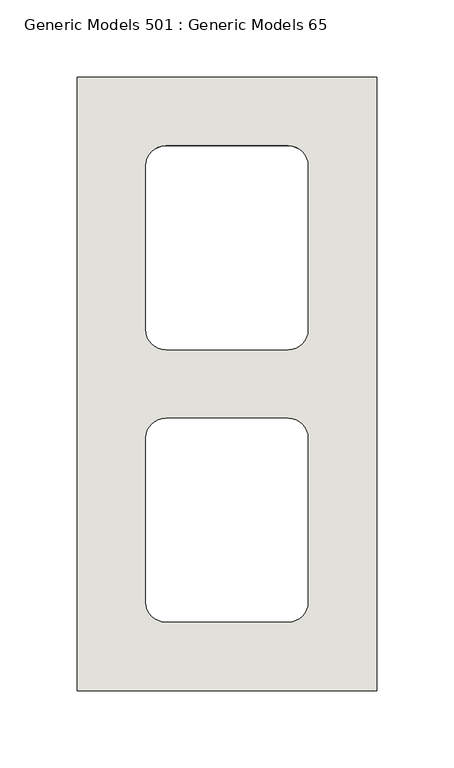
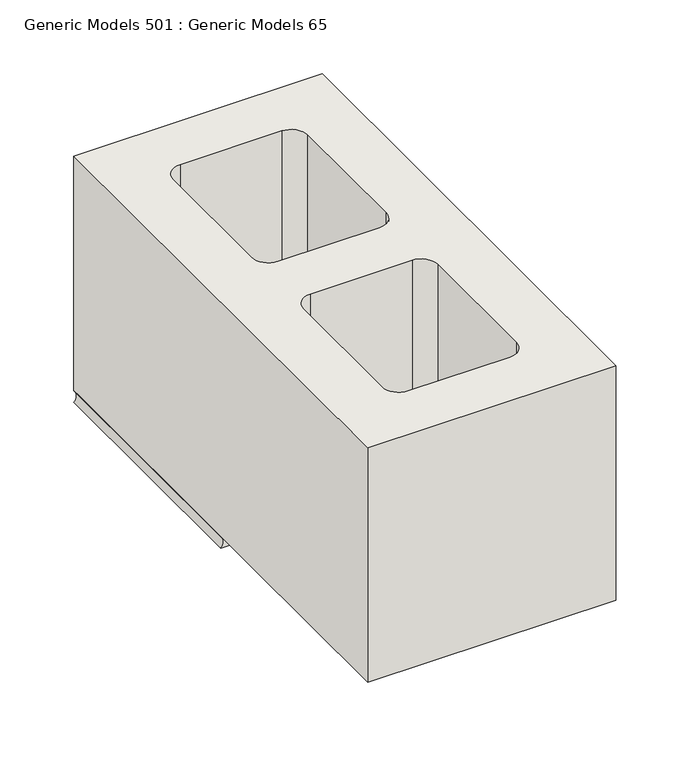
"""IFC4 building model written with IfcOpenShell, lengths in millimetres: wall geometry, Generic Models 501 : Generic Models 65."""

from ifc_helpers import new_model, si_unit, point, frame, frame_2d, origin, place, context, project, spatial, polyline, circle_curve, trimmed, segment, composite_curve, outline, extrude, source, transform, mapped, element, save
from ifc_brep_helpers import plane_surface, revolved_surface, advanced_brep


def generic_models_501_generic_models_65_e36d2a8f(model_context):
    return source(origin(), model_context, "Body", "SolidModel", [
        advanced_brep(
        [(428979.0125, 503.2375, 415.925), (428785.3375, 503.2375, 415.925), (428785.3375, 503.2375, 406.4), (428979.0125, 503.2375, 406.4), (428979.0125, 701.675, 415.925), (428979.0125, 701.675, 406.4), (428785.3375, 701.675, 406.4), (428785.3375, 701.675, 415.925), (428934.5625, 538.1625, 415.925), (428921.8625, 525.4625, 415.925), (428842.4875, 525.4625, 415.925), (428829.7875, 538.1625, 415.925), (428829.7875, 644.525, 415.925), (428842.4875, 657.225, 415.925), (428921.8625, 657.225, 415.925), (428934.5625, 644.525, 415.925), (428921.8625, 525.4625, 406.4), (428934.5625, 538.1625, 406.4), (428842.4875, 525.4625, 406.4), (428829.7875, 538.1625, 406.4), (428829.7875, 644.525, 406.4), (428842.4875, 657.225, 406.4), (428921.8625, 657.225, 406.4), (428934.5625, 644.525, 406.4)],
        [
            (0, 1),
            (1, 2, circle_curve(frame((428780.4545028, 503.2375, 411.1625), z_axis=(0.0, 1.0, 0.0), x_axis=(1.0, 0.0, 0.0)), 6.8209287)),
            (2, 3),
            (3, 0, circle_curve(frame((428983.8954972, 503.2375, 411.1625), z_axis=(0.0, 1.0, 0.0), x_axis=(-1.0, 0.0, 0.0)), 6.8209287)),
            (4, 5, circle_curve(frame((428983.8954972, 701.675, 411.1625), z_axis=(0.0, -1.0, 0.0), x_axis=(-1.0, 0.0, 0.0)), 6.8209287)),
            (5, 6),
            (6, 7, circle_curve(frame((428780.4545028, 701.675, 411.1625), z_axis=(0.0, -1.0, 0.0), x_axis=(1.0, 0.0, 0.0)), 6.8209287)),
            (7, 4),
            (0, 4),
            (7, 1),
            (8, 9, circle_curve(frame((428921.8625, 538.1625, 415.925), z_axis=(0.0, 0.0, -1.0), x_axis=(-1.0, 0.0, 0.0)), 12.7)),
            (9, 10),
            (10, 11, circle_curve(frame((428842.4875, 538.1625, 415.925), z_axis=(0.0, 0.0, -1.0), x_axis=(-1.0, 0.0, 0.0)), 12.7)),
            (11, 12),
            (12, 13, circle_curve(frame((428842.4875, 644.525, 415.925), z_axis=(0.0, 0.0, -1.0), x_axis=(-1.0, 0.0, 0.0)), 12.7)),
            (13, 14),
            (14, 15, circle_curve(frame((428921.8625, 644.525, 415.925), z_axis=(0.0, 0.0, -1.0), x_axis=(-1.0, 0.0, 0.0)), 12.7)),
            (15, 8),
            (16, 9),
            (8, 17),
            (17, 16, circle_curve(frame((428921.8625, 538.1625, 406.4), z_axis=(0.0, 0.0, -1.0), x_axis=(-1.0, 0.0, 0.0)), 12.7)),
            (16, 18),
            (18, 10),
            (18, 19, circle_curve(frame((428842.4875, 538.1625, 406.4), z_axis=(0.0, 0.0, -1.0), x_axis=(-1.0, 0.0, 0.0)), 12.7)),
            (19, 11),
            (19, 20),
            (20, 12),
            (20, 21, circle_curve(frame((428842.4875, 644.525, 406.4), z_axis=(0.0, 0.0, -1.0), x_axis=(-1.0, 0.0, 0.0)), 12.7)),
            (21, 13),
            (21, 22),
            (22, 14),
            (22, 23, circle_curve(frame((428921.8625, 644.525, 406.4), z_axis=(0.0, 0.0, -1.0), x_axis=(-1.0, 0.0, 0.0)), 12.7)),
            (23, 15),
            (23, 17),
            (6, 2),
            (5, 3),
        ],
        [
            plane_surface(frame((428882.175, 503.2375, 416.321875), z_axis=(0.0, -1.0, 0.0), x_axis=(0.0, 0.0, 1.0))),
            plane_surface(frame((428882.175, 701.675, 416.321875), z_axis=(0.0, 1.0, 0.0), x_axis=(0.0, 0.0, 1.0))),
            plane_surface(frame((428979.0125, 503.2375, 415.925), z_axis=(0.0, 0.0, 1.0), x_axis=(0.0, 1.0, 0.0))),
            revolved_surface(polyline([(428909.1625, 538.1625, 415.925), (428909.1625, 538.1625, 406.4)]), (428921.8625, 538.1625, 600.075), (0.0, 0.0, 1.0)),
            plane_surface(frame((428842.4875, 525.4625, 600.075), z_axis=(0.0, 1.0, 0.0), x_axis=(0.0, 0.0, -1.0))),
            revolved_surface(polyline([(428829.7875, 538.1625, 415.925), (428829.7875, 538.1625, 406.4)]), (428842.4875, 538.1625, 600.075), (0.0, 0.0, 1.0)),
            plane_surface(frame((428829.7875, 644.525, 600.075), z_axis=(1.0, 0.0, 0.0), x_axis=(0.0, 0.0, -1.0))),
            revolved_surface(polyline([(428829.7875, 644.525, 415.925), (428829.7875, 644.525, 406.4)]), (428842.4875, 644.525, 600.075), (0.0, 0.0, 1.0)),
            plane_surface(frame((428921.8625, 657.225, 600.075), z_axis=(0.0, -1.0, 0.0), x_axis=(0.0, 0.0, -1.0))),
            revolved_surface(polyline([(428909.1625, 644.525, 415.925), (428909.1625, 644.525, 406.4)]), (428921.8625, 644.525, 600.075), (0.0, 0.0, 1.0)),
            plane_surface(frame((428934.5625, 538.1625, 600.075), z_axis=(-1.0, 0.0, 0.0), x_axis=(0.0, 0.0, -1.0))),
            revolved_surface(polyline([(428787.2754315, 701.675, 411.1625), (428787.2754315, 503.2375, 411.1625)]), (428780.4545028, 503.2375, 411.1625), (0.0, 1.0, 0.0)),
            plane_surface(frame((428785.3375, 503.2375, 406.4), z_axis=(0.0, 0.0, -1.0), x_axis=(0.0, 1.0, 0.0))),
            revolved_surface(polyline([(428977.07456850004, 701.675, 411.1625), (428977.07456850004, 503.2375, 411.1625)]), (428983.8954972, 503.2375, 411.1625), (0.0, 1.0, 0.0)),
        ],
        [
            (0, [[1, 2, 3, 4]]),
            (1, [[5, 6, 7, 8]]),
            (2, [[-1, 9, -8, 10], [11, 12, 13, 14, 15, 16, 17, 18]]),
            (3, [[19, -11, 20, 21]]),
            (4, [[-19, 22, 23, -12]]),
            (5, [[-23, 24, 25, -13]]),
            (6, [[-25, 26, 27, -14]]),
            (7, [[-27, 28, 29, -15]]),
            (8, [[-29, 30, 31, -16]]),
            (9, [[-31, 32, 33, -17]]),
            (10, [[-33, 34, -20, -18]]),
            (11, [[-2, -10, -7, 35]]),
            (12, [[-3, -35, -6, 36], [-21, -34, -32, -30, -28, -26, -24, -22]]),
            (13, [[-4, -36, -5, -9]]),
        ],
    ),
        extrude(outline(polyline([(428979.0125, 304.8), (428785.3375, 304.8), (428785.3375, 701.675), (428979.0125, 701.675), (428979.0125, 304.8)]), holes=[composite_curve([segment(polyline([(428934.5625, 538.1625), (428934.5625, 644.525)]), True, "CONTINUOUS"), segment(trimmed(circle_curve(frame_2d((428921.8625, 644.525)), 12.7), [point((428934.5625, 644.525))], [point((428921.8625, 657.225))], True, "CARTESIAN"), True, "CONTINUOUS"), segment(polyline([(428921.8625, 657.225), (428842.4875, 657.225)]), True, "CONTINUOUS"), segment(trimmed(circle_curve(frame_2d((428842.4875, 644.525)), 12.7), [point((428842.4875, 657.225))], [point((428829.7875, 644.525))], True, "CARTESIAN"), True, "CONTINUOUS"), segment(polyline([(428829.7875, 644.525), (428829.7875, 538.1625)]), True, "CONTINUOUS"), segment(trimmed(circle_curve(frame_2d((428842.4875, 538.1625)), 12.7), [point((428829.7875, 538.1625))], [point((428842.4875, 525.4625))], True, "CARTESIAN"), True, "CONTINUOUS"), segment(polyline([(428842.4875, 525.4625), (428921.8625, 525.4625)]), True, "CONTINUOUS"), segment(trimmed(circle_curve(frame_2d((428921.8625, 538.1625)), 12.7), [point((428921.8625, 525.4625))], [point((428934.5625, 538.1625))], True, "CARTESIAN"), True, "CONTINUOUS")], self_intersect=False), composite_curve([segment(polyline([(428829.7875, 468.3125), (428829.7875, 361.95)]), True, "CONTINUOUS"), segment(trimmed(circle_curve(frame_2d((428842.4875, 361.95)), 12.7), [point((428829.7875, 361.95))], [point((428842.4875, 349.25))], True, "CARTESIAN"), True, "CONTINUOUS"), segment(polyline([(428842.4875, 349.25), (428921.8625, 349.25)]), True, "CONTINUOUS"), segment(trimmed(circle_curve(frame_2d((428921.8625, 361.95)), 12.7), [point((428921.8625, 349.25))], [point((428934.5625, 361.95))], True, "CARTESIAN"), True, "CONTINUOUS"), segment(polyline([(428934.5625, 361.95), (428934.5625, 468.3125)]), True, "CONTINUOUS"), segment(trimmed(circle_curve(frame_2d((428921.8625, 468.3125)), 12.7), [point((428934.5625, 468.3125))], [point((428921.8625, 481.0125))], True, "CARTESIAN"), True, "CONTINUOUS"), segment(polyline([(428921.8625, 481.0125), (428842.4875, 481.0125)]), True, "CONTINUOUS"), segment(trimmed(circle_curve(frame_2d((428842.4875, 468.3125)), 12.7), [point((428842.4875, 481.0125))], [point((428829.7875, 468.3125))], True, "CARTESIAN"), True, "CONTINUOUS")], self_intersect=False)]), frame((0.0, 0.0, 415.925), z_axis=(0.0, 0.0, 1.0), x_axis=(1.0, 0.0, 0.0)), (0.0, 0.0, 1.0), 193.675),
    ])


if __name__ == "__main__":
    model = new_model("IFC4")
    model_context = context("Model", 3, world=origin())
    ifc_project = project(units=[si_unit("LENGTHUNIT", "METRE", prefix="MILLI")], contexts=[model_context])
    site = spatial("IfcSite", under=ifc_project)
    building = spatial("IfcBuilding", under=site)
    placement = place(None, origin())
    generic_models_501_generic_models_65_shape = generic_models_501_generic_models_65_e36d2a8f(model_context)
    element("IfcWall", 1, ObjectType="Generic Models 501 : Generic Models 65", at=placement, inside=building, context=model_context, shape_type="MappedRepresentation", body=[
        mapped(generic_models_501_generic_models_65_shape, transform((0.0, 0.0, 0.0), x_axis=(1.0, 0.0, 0.0), y_axis=(0.0, 1.0, 0.0), z_axis=(0.0, 0.0, 1.0))),
    ])
    save(model, "model.ifc")

# Revit data of these elements
# Element 1 (IfcWall, "Generic Models 501 : Generic Models 65")
#   Materials on its faces: "CMU (SEE 'WALL TAG' FOR SIZE)", "MORTAR JOINT"
# Materials
#   "CMU (SEE 'WALL TAG' FOR SIZE)": class "Masonry", colour RGB 203 203 199, transparency 0, Description = "Concrete masonry units", Cost = 0
#   "MORTAR JOINT": class "Generic", colour RGB 120 120 120, transparency 0, Cost = 0
